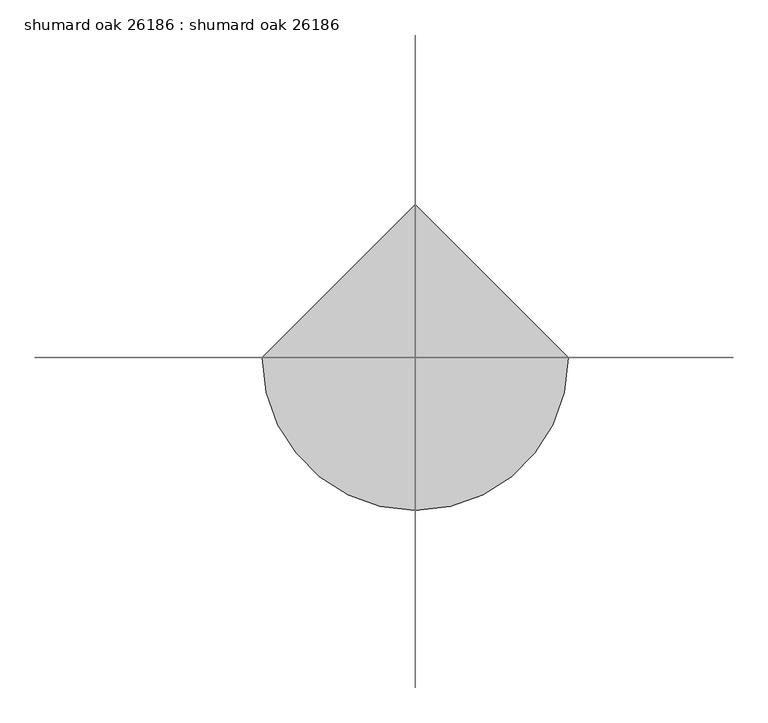
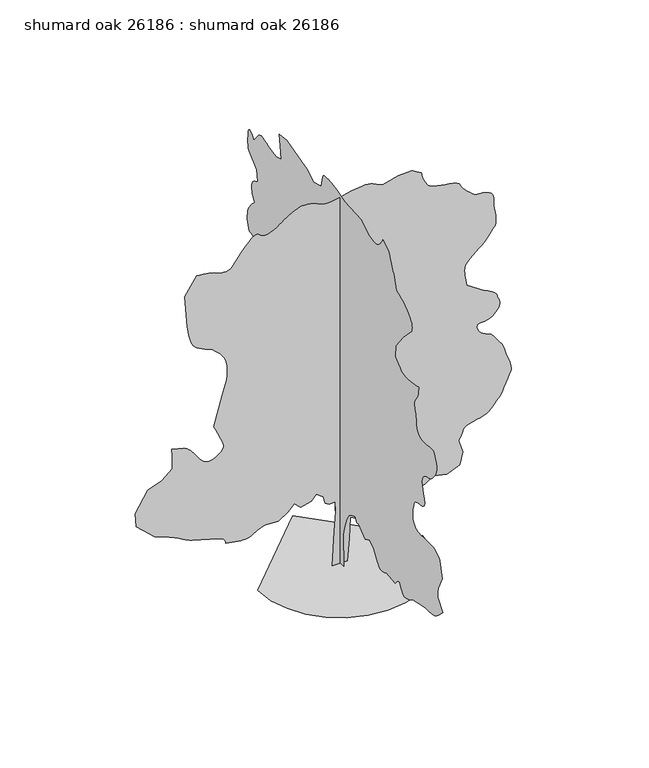
"""IFC4 building model written with IfcOpenShell, lengths in millimetres: proxy geometry, shumard oak 26186 : shumard oak 26186."""

import ifcopenshell
import ifcopenshell.guid

model = None  # the IFC model being written
_history = None  # IfcOwnerHistory: only IFC2X3 demands one
_inside = {}  # id of a spatial element -> (the spatial element, [elements in it])
_under = {}  # id of a project, library or spatial element -> (it, [spatial elements below it])
_declared = {}  # id of a project -> (the project, [libraries it declares])
_typed = {}  # id of a type object -> (the type object, [elements of that type])
_made_of = {}  # id of a material, layer set ... -> (it, [elements and type objects made of it])


def new_model(schema):
    """Start an empty IFC model of exactly this schema.

    Asked for "IFC4X3", IfcOpenShell would pick the latest addendum, in which some entities
    have other attributes; the version numbers below select the first issue.
    IFC2X3 requires an IfcOwnerHistory on every rooted entity: one is made here for all.
    """
    global model, _history
    if schema == "IFC4X3":
        model = ifcopenshell.file(schema_version=(4, 3, 0, 0))
    else:
        model = ifcopenshell.file(schema=schema)
    _inside.clear()
    _under.clear()
    _declared.clear()
    _typed.clear()
    _made_of.clear()
    _history = None
    if model.schema == "IFC2X3":
        org = make("IfcOrganization", Name="unknown")
        user = make(
            "IfcPersonAndOrganization",
            ThePerson=make("IfcPerson", FamilyName="unknown"),
            TheOrganization=org,
        )
        app = make(
            "IfcApplication",
            ApplicationDeveloper=org,
            Version="unknown",
            ApplicationFullName="unknown",
            ApplicationIdentifier="unknown",
        )
        _history = make(
            "IfcOwnerHistory",
            OwningUser=user,
            OwningApplication=app,
            ChangeAction="ADDED",
            CreationDate=0,
        )
    return model


def make(cls, **values):
    """One entity of the class cls with the attributes given. An attribute that is None is left unset."""
    return model.create_entity(
        cls, **{name: value for name, value in values.items() if value is not None}
    )


def rooted(cls, **values):
    """An entity with a GlobalId (a new one), such as an element, a storey or a relation."""
    return make(cls, GlobalId=ifcopenshell.guid.new(), OwnerHistory=_history, **values)


def si_unit(unit_type, name, prefix=None):
    """IfcSIUnit, for example si_unit("LENGTHUNIT", "METRE", prefix="MILLI")."""
    return make("IfcSIUnit", UnitType=unit_type, Prefix=prefix, Name=name)


def assignment(units):
    """IfcUnitAssignment: the units of a project."""
    return None if units is None else make("IfcUnitAssignment", Units=units)


def point(xyz):
    """IfcCartesianPoint."""
    return None if xyz is None else make("IfcCartesianPoint", Coordinates=xyz)


def direction(xyz):
    """IfcDirection."""
    return None if xyz is None else make("IfcDirection", DirectionRatios=xyz)


def frame(location, z_axis=None, x_axis=None):
    """IfcAxis2Placement3D, a coordinate frame: its origin and axes. An axis left out is left unset."""
    return make(
        "IfcAxis2Placement3D",
        Location=point(location),
        Axis=direction(z_axis),
        RefDirection=direction(x_axis),
    )


def origin():
    """The frame at (0, 0, 0) with its axes left unset."""
    return frame((0.0, 0.0, 0.0))


def place(relative_to, where):
    """IfcLocalPlacement: puts the frame where relative to a parent placement (None: the world)."""
    return make(
        "IfcLocalPlacement", PlacementRelTo=relative_to, RelativePlacement=where
    )


def context(
    kind, dimensions, precision=None, world=None, true_north=None, identifier=None
):
    """IfcGeometricRepresentationContext, for example the 3D "Model" context."""
    return make(
        "IfcGeometricRepresentationContext",
        ContextIdentifier=identifier,
        ContextType=kind,
        CoordinateSpaceDimension=dimensions,
        Precision=precision,
        WorldCoordinateSystem=world,
        TrueNorth=true_north,
    )


def project(units=None, contexts=None):
    """IfcProject with its units and contexts."""
    return rooted(
        "IfcProject",
        Name="project",
        RepresentationContexts=contexts,
        UnitsInContext=assignment(units),
    )


def spatial(cls, under=None, at=None, **own):
    """A site, building, storey or space (cls), placed at a placement, below another one or the project."""
    s = rooted(cls, ObjectPlacement=at, **own)
    if under is not None:
        _under.setdefault(under.id(), (under, []))[1].append(s)
    return s


def point_list(points):
    """IfcCartesianPointList2D or 3D."""
    cls = (
        "IfcCartesianPointList2D" if len(points[0]) == 2 else "IfcCartesianPointList3D"
    )
    return make(cls, CoordList=points)


def triangles(points, corners, closed=None, point_numbers=None):
    """IfcTriangulatedFaceSet: each triangle names its three corners, points numbered from 1."""
    return make(
        "IfcTriangulatedFaceSet",
        Coordinates=point_list(points),
        Closed=closed,
        CoordIndex=corners,
        PnIndex=point_numbers,
    )


def shape(context_of_items, identifier, shape_type, items):
    """IfcShapeRepresentation: the items that make up one representation, for example the "Body"."""
    return make(
        "IfcShapeRepresentation",
        ContextOfItems=context_of_items,
        RepresentationIdentifier=identifier,
        RepresentationType=shape_type,
        Items=items,
    )


def source(mapping_origin, context_of_items, identifier, shape_type, items):
    """IfcRepresentationMap: a shape defined once, which mapped items show again and again."""
    return make(
        "IfcRepresentationMap",
        MappingOrigin=mapping_origin,
        MappedRepresentation=shape(context_of_items, identifier, shape_type, items),
    )


def transform(
    local_origin,
    x_axis=None,
    y_axis=None,
    z_axis=None,
    scale=None,
    scale2=None,
    scale3=None,
    uniform=True,
):
    """IfcCartesianTransformationOperator3D, or its non-uniform kind. x_axis, y_axis, z_axis: its Axis1, 2, 3."""
    if uniform:
        return make(
            "IfcCartesianTransformationOperator3D",
            Axis1=direction(x_axis),
            Axis2=direction(y_axis),
            LocalOrigin=point(local_origin),
            Scale=scale,
            Axis3=direction(z_axis),
        )
    return make(
        "IfcCartesianTransformationOperator3DnonUniform",
        Axis1=direction(x_axis),
        Axis2=direction(y_axis),
        LocalOrigin=point(local_origin),
        Scale=scale,
        Axis3=direction(z_axis),
        Scale2=scale2,
        Scale3=scale3,
    )


def mapped(mapping_source, mapping_target):
    """IfcMappedItem: shows the shape of a source again, moved by a transform."""
    return make(
        "IfcMappedItem", MappingSource=mapping_source, MappingTarget=mapping_target
    )


def made_of(thing, what):
    """Note that an element or type object is made of a material, layer set ...; save() writes the relation."""
    if what is not None:
        _made_of.setdefault(what.id(), (what, []))[1].append(thing)
    return thing


def element(
    cls,
    number,
    at=None,
    inside=None,
    cuts=None,
    type_object=None,
    material=None,
    context=None,
    identifier="Body",
    shape_type=None,
    held_by="IfcProductDefinitionShape",
    body=None,
    shapes=None,
    **own,
):
    """One element of the class cls, such as IfcWall. Its Tag is "e" and its number.

    at: its placement. inside: the storey or other place that contains it. cuts: it is an
    opening in that element (IfcRelVoidsElement). A single representation is given by context,
    identifier, shape_type and body (its items); several are given by shapes. held_by: the class
    of the entity that holds the representations. save() writes the other relations.
    """
    e = rooted(cls, Tag="e%d" % number, ObjectPlacement=at, **own)
    if body is not None:
        shapes = [shape(context, identifier, shape_type, body)]
    if shapes is not None:
        e.Representation = make(held_by, Representations=shapes)
    if inside is not None:
        _inside.setdefault(inside.id(), (inside, []))[1].append(e)
    if cuts is not None:
        rooted(
            "IfcRelVoidsElement", RelatingBuildingElement=cuts, RelatedOpeningElement=e
        )
    if type_object is not None:
        _typed.setdefault(type_object.id(), (type_object, []))[1].append(e)
    return made_of(e, material)


def aggregate(whole, parts):
    """IfcRelAggregates: a whole, such as a stair, and the parts it consists of."""
    return rooted("IfcRelAggregates", RelatingObject=whole, RelatedObjects=parts)


def save(model, path):
    """Write the relations noted so far, then the file.

    IfcRelAggregates (storeys below a building ...), IfcRelContainedInSpatialStructure (elements
    in a storey), IfcRelDefinesByType, IfcRelAssociatesMaterial and IfcRelDeclares: one each for
    every whole, place, type object, material and project.
    """
    for whole, parts in _under.values():
        aggregate(whole, parts)
    for where, things in _inside.values():
        rooted(
            "IfcRelContainedInSpatialStructure",
            RelatedElements=things,
            RelatingStructure=where,
        )
    for kind, things in _typed.values():
        rooted("IfcRelDefinesByType", RelatedObjects=things, RelatingType=kind)
    for what, things in _made_of.values():
        rooted("IfcRelAssociatesMaterial", RelatedObjects=things, RelatingMaterial=what)
    for by, libraries in _declared.values():
        rooted("IfcRelDeclares", RelatingContext=by, RelatedDefinitions=libraries)
    model.write(path)


def shumard_oak_26186_shumard_oak_26186_cf07c7db(model_context):
    return source(origin(), model_context, "Body", "Tessellation", [
        triangles([(-0.0016958, 164.6246354, 0.0086022), (-0.0016958, -151.6104316, 0.0086022), (-0.0016958, -124.1113561, 783.7227293), (-0.0016958, -179.1089983, 1017.4612965), (-0.0016958, -261.6049622, 1237.4509209), (-0.0016958, -357.8507226, 1388.6927067), (-0.0016958, -467.8454985, 1457.4403999), (-0.0016958, -605.3383779, 1512.436607), (-0.0016958, -660.3370193, 1388.6927067), (-0.0016958, -756.5828161, 1416.1908829), (-0.0016958, -866.5775557, 1306.195998), (-0.0016958, -1017.8194868, 1209.9502739), (-0.0016958, -1196.5619196, 1292.4469826), (-0.0016958, -1361.5527935, 1182.452243), (-0.0016958, -1471.5476784, 989.9607222), (-0.0016958, -1498.1643677, 951.9597713), (-0.0016958, -1525.3829098, 915.7621988), (-0.0016958, -1553.8031227, 883.1739264), (-0.0016958, -1584.0290394, 855.9959341), (-0.0016958, -1616.658007, 836.0340712), (-0.0016958, -1652.2942039, 825.0891724), (-0.0016958, -1691.5371574, 824.9697756), (-0.0016958, -1729.1774471, 831.662681), (-0.0016958, -1760.3255459, 839.8008471), (-0.0016958, -1786.0582775, 849.1404659), (-0.0016958, -1807.4654011, 859.4426714), (-0.0016958, -1825.6238857, 870.4663445), (-0.0016958, -1841.6182583, 881.9725462), (-0.0016958, -1856.5307201, 893.7149254), (-0.0016958, -2214.0131149, 852.4678791), (-0.0016958, -2249.2480282, 893.1561659), (-0.0016958, -2283.7616192, 930.4738735), (-0.0016958, -2316.8324203, 961.0605967), (-0.0016958, -2347.7391094, 981.54314), (-0.0016958, -2375.7578934, 988.5586275), (-0.0016958, -2400.1697754, 978.7389507), (-0.0016958, -2420.2535786, 948.7136032), (-0.0016958, -2440.416156, 905.5412384), (-0.0016958, -2465.389341, 860.9260838), (-0.0016958, -2494.9323051, 818.4750412), (-0.0016958, -2528.8058189, 781.7974108), (-0.0016958, -2566.7735596, 754.4999491), (-0.0016958, -2608.5820541, 740.1896307), (-0.0016958, -2653.9973053, 742.4730669), (-0.0016958, -2699.5395836, 755.8614212), (-0.0016958, -2742.1861084, 772.1352098), (-0.0016958, -2782.4196991, 790.8169184), (-0.0016958, -2820.7484642, 811.421402), (-0.0016958, -2857.6293526, 833.4686754), (-0.0016958, -2893.5448929, 856.475992), (-0.0016958, -2928.9779045, 879.96591), (-0.0016958, -3423.9482735, 976.2117067), (-0.0016958, -3485.6956673, 976.3335743), (-0.0016958, -3546.579451, 977.174366), (-0.0016958, -3605.7868835, 979.4603456), (-0.0016958, -3662.4543549, 983.9078939), (-0.0016958, -3715.7688332, 991.2459635), (-0.0016958, -3764.8925789, 1002.1882462), (-0.0016958, -3808.9361115, 1017.4612965), (-0.0016958, -3851.3797417, 1039.546649), (-0.0016958, -3896.0075409, 1069.5719965), (-0.0016958, -3942.4134293, 1106.2115479), (-0.0016958, -3990.2924835, 1148.1393665), (-0.0016958, -4039.2383331, 1194.0371464), (-0.0016958, -4088.8951859, 1242.5817123), (-0.0016958, -4138.9334106, 1292.4469826), (-0.0016958, -3946.4265564, 1512.436607), (-0.0016958, -3940.7114983, 1553.6455742), (-0.0016958, -3935.9362083, 1594.6132771), (-0.0016958, -3933.0916145, 1635.0983059), (-0.0016958, -3933.1169037, 1674.8646286), (-0.0016958, -3937.0032944, 1713.6657486), (-0.0016958, -3945.7152626, 1751.2679592), (-0.0016958, -3960.1934486, 1787.4247639), (-0.0016958, -4111.425206, 2103.6601124), (-0.0016958, -4015.1842781, 2488.640538), (-0.0016958, -4007.6405525, 2499.2628548), (-0.0016958, -3985.1869812, 2526.4815422), (-0.0016958, -3948.0776184, 2563.3191193), (-0.0016958, -3896.5156494, 2602.8164177), (-0.0016958, -3830.780127, 2637.9697952), (-0.0016958, -3751.1003975, 2661.820665), (-0.0016958, -3657.7046448, 2667.3831161), (-0.0016958, -3553.6406479, 2663.0650658), (-0.0016958, -3446.4524231, 2661.3634254), (-0.0016958, -3343.1000107, 2661.617189), (-0.0016958, -3250.5928665, 2663.0650658), (-0.0016958, -3175.8660324, 2664.970182), (-0.0016958, -3125.9298363, 2666.6718224), (-0.0016958, -3107.7178665, 2667.3831161), (-0.0016958, -3097.049913, 2674.6474983), (-0.0016958, -3069.5669975, 2695.1200859), (-0.0016958, -3031.9495262, 2726.9207611), (-0.0016958, -2990.9793526, 2768.0688309), (-0.0016958, -2953.3874611, 2816.7097572), (-0.0016958, -2925.9045456, 2870.8625565), (-0.0016958, -2915.2365921, 2928.622403), (-0.0016958, -2917.2431557, 2986.3310898), (-0.0016958, -2922.8564758, 3041.9064766), (-0.0016958, -2931.4672874, 3095.6529053), (-0.0016958, -2942.4907425, 3147.977037), (-0.0016958, -2955.3178665, 3199.2087936), (-0.0016958, -2969.3385223, 3249.7039673), (-0.0016958, -2983.9690247, 3299.8436394), (-0.0016958, -2996.0086967, 3314.52472), (-0.0016958, -3009.4706657, 3328.8250099), (-0.0016958, -3025.8280975, 3342.414006), (-0.0016958, -3046.5038704, 3354.9362068), (-0.0016958, -3072.9705688, 3365.9852417), (-0.0016958, -3106.6510712, 3375.2561874), (-0.0016958, -3148.9673836, 3382.3429642), (-0.0016958, -3200.1485619, 3386.6863037), (-0.0016958, -3255.4443146, 3391.740937), (-0.0016958, -3308.7843727, 3403.2725006), (-0.0016958, -3354.1996239, 3427.0722107), (-0.0016958, -3385.6703773, 3468.9315742), (-0.0016958, -3397.1766518, 3534.5906479), (-0.0016958, -3382.6984657, 3629.8406479), (-0.0016958, -3353.0819595, 3737.5114014), (-0.0016958, -3325.8786781, 3836.2667107), (-0.0016958, -3305.152327, 3925.6746254), (-0.0016958, -3294.9921913, 4005.2023293), (-0.0016958, -3299.5387161, 4074.3920013), (-0.0016958, -3322.8306084, 4132.761113), (-0.0016958, -3368.9571533, 4179.8018463), (-0.0016958, -3425.5228867, 4212.7710548), (-0.0016958, -3477.9993347, 4232.964299), (-0.0016958, -3527.3262657, 4246.1975029), (-0.0016958, -3574.5193153, 4258.2118858), (-0.0016958, -3620.493544, 4274.8233719), (-0.0016958, -3666.2390076, 4301.7473099), (-0.0016958, -3712.6954742, 4344.8004959), (-0.0016958, -3760.0411308, 4399.562851), (-0.0016958, -3805.2023277, 4457.9322533), (-0.0016958, -3844.3694138, 4520.1368866), (-0.0016958, -3873.6809967, 4586.4308052), (-0.0016958, -3889.2765564, 4657.068354), (-0.0016958, -3887.295282, 4732.2777168), (-0.0016958, -3863.9272316, 4812.2879494), (-0.0016958, -3835.7077332, 4887.9545517), (-0.0016958, -3816.632444, 4949.7019455), (-0.0016958, -3799.0047409, 4996.9967331), (-0.0016958, -3775.1032928, 5029.3819656), (-0.0016958, -3737.2573471, 5046.3745331), (-0.0016958, -3677.7705711, 5047.4919067), (-0.0016958, -3588.9466324, 5032.2771378), (-0.0016958, -3483.5620766, 5015.437468), (-0.0016958, -3382.266806, 5012.0591858), (-0.0016958, -3289.150106, 5022.1684525), (-0.0016958, -3208.3018433, 5045.7396881), (-0.0016958, -3143.7860138, 5082.7728928), (-0.0016958, -3099.7421906, 5133.2930649), (-0.0016958, -3080.2096619, 5197.2507889), (-0.0016958, -3073.5295464, 5265.5768509), (-0.0016958, -3065.4015541, 5329.5339935), (-0.0016958, -3056.0541595, 5389.9099594), (-0.0016958, -3045.7417076, 5447.3901718), (-0.0016958, -3034.7182526, 5502.7112137), (-0.0016958, -3023.2119781, 5556.5846695), (-0.0016958, -3011.4772293, 5609.7471222), (-0.0016958, -3000.047113, 5648.0755966), (-0.0016958, -2990.8014565, 5686.505809), (-0.0016958, -2985.8485611, 5725.1900757), (-0.0016958, -2987.423465, 5764.2295532), (-0.0016958, -2997.6341789, 5803.7521408), (-0.0016958, -3018.6907425, 5843.8839935), (-0.0016958, -3052.7267464, 5884.7274307), (-0.0016958, -3089.125106, 5934.8418137), (-0.0016958, -3116.6080215, 5997.6815826), (-0.0016958, -3136.4198936, 6065.8297485), (-0.0016958, -3149.7295464, 6131.8187439), (-0.0016958, -3157.7558006, 6188.1815826), (-0.0016958, -3161.6674805, 6227.450116), (-0.0016958, -3162.7089867, 6242.2073547), (-0.0016958, -3142.4395844, 6237.6861191), (-0.0016958, -3088.0074417, 6226.1798447), (-0.0016958, -3009.0387154, 6210.8383392), (-0.0016958, -2915.160434, 6194.7602509), (-0.0016958, -2815.9731743, 6181.0948059), (-0.0016958, -2721.1295448, 6172.9418152), (-0.0016958, -2640.2304131, 6173.4749222), (-0.0016958, -2571.9299309, 6185.3619873), (-0.0016958, -2507.9599983, 6208.094902), (-0.0016958, -2447.5915901, 6239.8452896), (-0.0016958, -2390.1089069, 6278.808609), (-0.0016958, -2334.7901905, 6323.1826447), (-0.0016958, -2280.9167347, 6371.1634369), (-0.0016958, -2227.7621304, 6420.9476074), (-0.0016958, -2241.5111458, 6709.6945175), (-0.0016958, -2543.9897758, 7094.6826462), (-0.0016958, -2887.7283875, 7452.1625702), (-0.0016958, -2893.1132332, 7496.4860275), (-0.0016958, -2895.3482712, 7541.6722229), (-0.0016958, -2891.335144, 7588.5356415), (-0.0016958, -2877.9493332, 7637.9128601), (-0.0016958, -2852.0666107, 7690.6689423), (-0.0016958, -2810.5377502, 7747.6160477), (-0.0016958, -2750.2379425, 7809.6424942), (-0.0016958, -2679.5242355, 7869.2562973), (-0.0016958, -2608.8108192, 7919.4724182), (-0.0016958, -2538.10467, 7961.8901779), (-0.0016958, -2467.3935791, 7998.0344833), (-0.0016958, -2396.6824883, 8029.5052368), (-0.0016958, -2325.9712521, 8057.8517624), (-0.0016958, -2255.2601612, 8084.6233841), (-0.0016958, -2234.6175259, 8155.1336151), (-0.0016958, -2213.8530956, 8224.4503143), (-0.0016958, -2192.8472557, 8291.3537888), (-0.0016958, -2171.4808273, 8354.651088), (-0.0016958, -2149.6341957, 8413.1219376), (-0.0016958, -2127.1881821, 8465.5983856), (-0.0016958, -2104.0183754, 8510.8607391), (-0.0016958, -2078.3235775, 8560.2129593), (-0.0016958, -2049.9822842, 8621.0970337), (-0.0016958, -2021.4021973, 8686.5529221), (-0.0016958, -1994.9862225, 8749.5955856), (-0.0016958, -1973.1395908, 8803.2917267), (-0.0016958, -1958.2679695, 8840.6039841), (-0.0016958, -1952.7738281, 8854.5996414), (-0.0016958, -1719.0353336, 8992.089505), (-0.0016958, -1707.0516174, 8968.3915329), (-0.0016958, -1693.863905, 8943.9819763), (-0.0016958, -1678.2681999, 8918.1248337), (-0.0016958, -1659.0683544, 8890.1085205), (-0.0016958, -1635.057756, 8859.1970352), (-0.0016958, -1605.0324085, 8824.678212), (-0.0016958, -1567.7934025, 8785.841629), (-0.0016958, -1522.9369835, 8752.2122864), (-0.0016958, -1471.5882282, 8732.2983856), (-0.0016958, -1414.8268673, 8723.7896027), (-0.0016958, -1353.7372822, 8724.4244476), (-0.0016958, -1289.3990582, 8731.9175949), (-0.0016958, -1222.896722, 8743.9825562), (-0.0016958, -1155.3123299, 8758.3334244), (-0.0016958, -852.8259968, 8964.5813004), (-0.0016958, -192.8582863, 9005.8311081), (-0.0016958, -107.5965211, 9029.2756073), (-0.0016958, -23.416737, 9052.008522), (-0.0016958, 58.5983536, 9073.2938507), (-0.0016958, 137.366361, 9092.4200089), (-0.0016958, 211.8051857, 9108.6504135), (-0.0016958, 280.8327856, 9121.2740616), (-0.0016958, 343.3650879, 9129.57995), (-0.0016958, 405.0185557, 9135.9045639), (-0.0016958, 469.5549508, 9141.5181747), (-0.0016958, 533.1311937, 9144.0075577), (-0.0016958, 591.8966838, 9140.9594879), (-0.0016958, 642.0033274, 9129.9863205), (-0.0016958, 679.6029219, 9108.6504135), (-0.0016958, 700.8500261, 9074.5891205), (-0.0016958, 769.5952486, 8799.5832321), (-0.0016958, 1072.081509, 8717.1091965), (-0.0016958, 1347.0698112, 8882.0822662), (-0.0016958, 1690.8031906, 8964.5813004), (-0.0016958, 2144.5313095, 9102.0717453), (-0.0016958, 2447.0174973, 9060.8225189), (-0.0016958, 2419.5169956, 8799.5832321), (-0.0016958, 2364.5209339, 8497.1197174), (-0.0016958, 2584.5030006, 8428.361705), (-0.0016958, 2804.4924797, 8469.6115128), (-0.0016958, 2889.5570549, 8501.5647949), (-0.0016958, 2972.3357231, 8530.7490601), (-0.0016958, 3050.5425774, 8554.3964539), (-0.0016958, 3121.8911293, 8569.7385406), (-0.0016958, 3184.1210518, 8574.0307205), (-0.0016958, 3234.8958595, 8564.480722), (-0.0016958, 3271.9799332, 8538.3439453), (-0.0016958, 3478.2280998, 8290.8712601), (-0.0016958, 3525.090937, 8345.6591949), (-0.0016958, 3570.2521339, 8393.3603531), (-0.0016958, 3612.0606285, 8426.8885391), (-0.0016958, 3648.8144897, 8439.1058167), (-0.0016958, 3678.8373665, 8422.9515701), (-0.0016958, 3700.4526169, 8371.313443), (-0.0016958, 3711.9588913, 8277.1046585), (-0.0016958, 3715.4389114, 8172.4819748), (-0.0016958, 3714.6005905, 8091.684581), (-0.0016958, 3710.155513, 8030.6987686), (-0.0016958, 3702.8149727, 7985.6137299), (-0.0016958, 3693.3152618, 7952.4163376), (-0.0016958, 3682.3679649, 7927.1684601), (-0.0016958, 3670.7093742, 7905.8831314), (-0.0016958, 3354.4789673, 7644.6438446), (-0.0016958, 3326.9707626, 7355.921933), (-0.0016958, 3370.9384277, 7337.989888), (-0.0016958, 3413.6102417, 7318.6346741), (-0.0016958, 3453.615358, 7296.384288), (-0.0016958, 3489.6326363, 7269.8161423), (-0.0016958, 3520.3920959, 7237.4564896), (-0.0016958, 3544.5220184, 7197.8833237), (-0.0016958, 3560.7018448, 7149.674057), (-0.0016958, 3566.8994316, 7096.6389221), (-0.0016958, 3562.9624626, 7043.6032059), (-0.0016958, 3550.618158, 6990.568071), (-0.0016958, 3531.5425781, 6937.5329361), (-0.0016958, 3507.4126556, 6884.4978012), (-0.0016958, 3479.904451, 6831.4626663), (-0.0016958, 3450.7198952, 6778.4269501), (-0.0016958, 3494.7381386, 6734.2313919), (-0.0016958, 3537.6640068, 6689.8829361), (-0.0016958, 3578.4309952, 6645.3060059), (-0.0016958, 3615.9470192, 6600.3732834), (-0.0016958, 3649.1447021, 6554.9580322), (-0.0016958, 3676.9322502, 6508.9329346), (-0.0016958, 3698.2175789, 6462.1968338), (-0.0016958, 3713.4829262, 6416.6548462), (-0.0016958, 3724.4305138, 6374.0080307), (-0.0016958, 3731.7710541, 6333.77444), (-0.0016958, 3736.2161316, 6295.4459656), (-0.0016958, 3738.5020386, 6258.5650772), (-0.0016958, 3739.3400688, 6222.6492462), (-0.0016958, 3739.4670959, 6187.2165253), (-0.0016958, 3656.9680618, 5953.4854431), (-0.0016958, 3618.6901657, 5947.3387253), (-0.0016958, 3580.5140076, 5939.7694199), (-0.0016958, 3542.591613, 5929.304361), (-0.0016958, 3505.0250107, 5914.5215424), (-0.0016958, 3467.9665169, 5893.9477982), (-0.0016958, 3431.4664192, 5866.1599594), (-0.0016958, 3395.728775, 5829.7366013), (-0.0016958, 3363.165937, 5786.4799393), (-0.0016958, 3335.6830215, 5739.6171021), (-0.0016958, 3312.3911293, 5689.7567734), (-0.0016958, 3292.4522301, 5637.4838013), (-0.0016958, 3275.0532921, 5583.4068695), (-0.0016958, 3259.3559944, 5528.1364059), (-0.0016958, 3244.4717285, 5472.2566772), (-0.0016958, 3212.2896812, 5428.0349579), (-0.0016958, 3181.4287743, 5383.7120819), (-0.0016958, 3153.2092758, 5339.1351517), (-0.0016958, 3128.9523262, 5294.1768494), (-0.0016958, 3110.0037735, 5248.7615982), (-0.0016958, 3097.6341797, 5202.7620804), (-0.0016958, 3093.2399712, 5156.026561), (-0.0016958, 3106.9812836, 4784.7797447), (-0.0016958, 3139.1630402, 4781.5284897), (-0.0016958, 3170.049527, 4776.4738564), (-0.0016958, 3198.2690254, 4767.8377556), (-0.0016958, 3222.5006859, 4753.7662308), (-0.0016958, 3241.4745277, 4732.4809021), (-0.0016958, 3253.8188324, 4702.1533928), (-0.0016958, 3258.2383301, 4661.0306122), (-0.0016958, 3257.0192184, 4613.5073502), (-0.0016958, 3253.6665161, 4565.2219254), (-0.0016958, 3248.4848557, 4516.377523), (-0.0016958, 3241.8808983, 4467.0253029), (-0.0016958, 3234.1845657, 4417.3175812), (-0.0016958, 3225.7516502, 4367.3810944), (-0.0016958, 3216.988813, 4317.2922913), (-0.0016958, 3203.2219208, 4042.311692), (-0.0016958, 3464.4612076, 4056.0785843), (-0.0016958, 3753.208699, 4111.0694138), (-0.0016958, 3814.6511696, 4090.2669044), (-0.0016958, 3873.5792587, 4068.37202), (-0.0016958, 3927.4527145, 4044.3182556), (-0.0016958, 3973.7568649, 4017.0132362), (-0.0016958, 4009.9520393, 3985.3901665), (-0.0016958, 4033.523275, 3948.3569618), (-0.0016958, 4041.9306107, 3904.8212471), (-0.0016958, 4039.5429657, 3849.6778107), (-0.0016958, 4032.8119812, 3780.081768), (-0.0016958, 4022.448951, 3698.4716331), (-0.0016958, 4009.2407455, 3607.2347603), (-0.0016958, 3993.8483711, 3508.7840836), (-0.0016958, 3977.00812, 3405.5078293), (-0.0016958, 3959.4568657, 3299.8436394), (-0.0016958, 3835.7077332, 2969.87192), (-0.0016958, 3768.1185448, 2931.9498161), (-0.0016958, 3701.6211502, 2896.3136192), (-0.0016958, 3637.2829262, 2865.2492363), (-0.0016958, 3576.1959572, 2841.0431557), (-0.0016958, 3519.4267479, 2825.9554138), (-0.0016958, 3468.0679642, 2822.3233681), (-0.0016958, 3423.2113998, 2832.3817657), (-0.0016958, 3038.248851, 2997.3548355), (-0.0016958, 2653.2607224, 2873.6312828), (-0.0016958, 2378.2699493, 2681.1244286), (-0.0016958, 2103.2842632, 2268.651059), (-0.0016958, 2076.6675739, 2227.6428062), (-0.0016958, 2049.4488865, 2188.0796688), (-0.0016958, 2021.0263481, 2151.4021111), (-0.0016958, 1990.8027569, 2119.0526321), (-0.0016958, 1958.1739346, 2092.4764927), (-0.0016958, 1922.5377377, 2073.1141571), (-0.0016958, 1883.2946388, 2062.4105953), (-0.0016958, 1844.1303143, 2058.8443886), (-0.0016958, 1807.3715115, 2059.123732), (-0.0016958, 1770.371299, 2062.0498615), (-0.0016958, 1730.4881229, 2066.4186356), (-0.0016958, 1685.070401, 2071.0288193), (-0.0016958, 1631.4762886, 2074.6762711), (-0.0016958, 1567.0592903, 2076.1596107), (-0.0016958, 1497.9510086, 2070.950045), (-0.0016958, 1431.730632, 2056.3577671), (-0.0016958, 1367.9130157, 2033.9498325), (-0.0016958, 1306.020718, 2005.2883553), (-0.0016958, 1245.5712101, 1971.9382107), (-0.0016958, 1186.0844341, 1935.4612221), (-0.0016958, 1127.0801868, 1897.4196487), (-0.0016958, 1044.5834782, 1663.6810089), (-0.0016958, 810.8448383, 1402.4418674), (-0.0016958, 778.5741337, 1367.4862976), (-0.0016958, 741.256426, 1333.2546661), (-0.0016958, 699.7273476, 1299.622562), (-0.0016958, 654.8303061, 1266.4729866), (-0.0016958, 607.408455, 1233.6815289), (-0.0016958, 558.3051295, 1201.1339516), (-0.0016958, 508.3585416, 1168.7032276), (-0.0016958, 425.8618329, 1457.4403999), (-0.0016958, 288.3689717, 1649.9293774), (-0.0016958, 233.3715837, 1526.1856224), (-0.0016958, 192.1232112, 1333.696645), (-0.0016958, 178.3741776, 989.9607222), (-0.0016958, 150.8753565, 508.7344634), (170.3625119, 0.000436, 0.0217742), (-187.1199193, 0.000436, 0.0217742), (-132.1230309, 0.000387, 824.9824928), (-104.6242098, 0.0003581, 1306.2087879), (-118.3734886, 0.0003434, 1553.698914), (-255.8671038, 0.0003442, 1539.9498985), (-352.1128461, 0.000341, 1594.9459602), (-393.359965, 0.0003302, 1773.6885384), (-558.3534187, 0.0003237, 1883.6832779), (-668.3482309, 0.000331, 1759.9395229), (-915.8358135, 0.0003352, 1691.1918297), (-1067.0802881, 0.0003271, 1828.6846001), (-1218.3221466, 0.000336, 1677.4428143), (-1438.311771, 0.0003442, 1539.9498985), (-1768.2961349, 0.0003434, 1553.698914), (-1933.2869362, 0.0003476, 1484.9512207), (-1968.7250347, 0.0003491, 1458.6138748), (-2004.6407204, 0.0003507, 1433.3612011), (-2041.5189926, 0.000352, 1410.2726395), (-2079.8425255, 0.0003531, 1390.4301006), (-2120.0889061, 0.0003541, 1374.915786), (-2162.738047, 0.0003547, 1364.8142223), (-2208.2752384, 0.0003549, 1361.2074657), (-2259.0244663, 0.0003549, 1362.8101295), (-2316.2658852, 0.0003547, 1367.3008438), (-2378.9175842, 0.0003541, 1374.1944637), (-2445.902449, 0.0003536, 1383.0132568), (-2516.1310112, 0.0003531, 1393.2749851), (-2588.5161278, 0.0003523, 1404.4991547), (-2661.9982704, 0.0003518, 1416.2061436), (-2665.4018417, 0.0003499, 1445.5887978), (-2671.5741394, 0.0003481, 1474.4889233), (-2683.2835991, 0.0003465, 1502.428933), (-2703.2986565, 0.0003449, 1528.9262981), (-2734.3630394, 0.0003434, 1553.4981995), (-2779.2448929, 0.0003421, 1575.6648697), (-2840.7382324, 0.000341, 1594.9459602), (-3445.7158401, 0.0003302, 1773.6885384), (-3495.0936401, 0.0003295, 1789.3602562), (-3547.8494316, 0.0003281, 1811.5293972), (-3602.2815742, 0.0003266, 1838.265556), (-3656.7140076, 0.0003247, 1867.6482101), (-3709.469799, 0.0003229, 1897.7523319), (-3758.8728882, 0.0003213, 1926.6550735), (-3803.1957642, 0.0003197, 1952.4285004), (-3850.8716331, 0.0003182, 1977.2011162), (-3910.0790657, 0.0003166, 2004.1403149), (-3978.8876564, 0.0003148, 2032.8804211), (-4055.4181595, 0.0003132, 2063.0657879), (-4137.7140083, 0.0003113, 2094.3332108), (-4223.8456696, 0.0003092, 2126.3194851), (-4311.9327347, 0.0003074, 2158.668964), (-4738.1450912, 0.0002835, 2557.4011665), (-4765.6532959, 0.0002638, 2887.3725952), (-4476.9060951, 0.000236, 3354.8600487), (-4146.9343758, 0.0002287, 3478.6088905), (-3899.4364014, 0.0002163, 3684.8570572), (-3899.4364014, 0.0001977, 4001.0874641), (-3913.2032936, 0.0001877, 4166.0858231), (-3624.4558022, 0.0001919, 4097.3281013), (-3591.9438332, 0.0001932, 4076.3729851), (-3558.8475975, 0.0001945, 4053.3607269), (-3524.5322502, 0.0001961, 4026.2588928), (-3488.4135246, 0.0001979, 3993.03563), (-3449.8815742, 0.0002006, 3951.6082169), (-3408.3524231, 0.0002037, 3899.9953789), (-3363.216806, 0.0002074, 3836.0888145), (-3317.4713425, 0.0002113, 3768.956575), (-3273.4275192, 0.000215, 3709.7491425), (-3229.3839867, 0.0002179, 3659.6856285), (-3183.6385231, 0.0002203, 3619.9601463), (-3134.5403572, 0.0002221, 3591.765937), (-3080.387558, 0.0002229, 3576.3482735), (-3019.4781944, 0.0002229, 3574.8495277), (-2952.9046417, 0.0002221, 3590.0895859), (-2885.848851, 0.0002203, 3620.9507835), (-2822.8567657, 0.0002176, 3662.8860146), (-2768.5513596, 0.0002147, 3711.2984665), (-2727.4541588, 0.0002119, 3761.6413239), (-2704.1622665, 0.000209, 3809.3427727), (-2703.2480782, 0.0002066, 3849.8304176), (-2719.4531937, 0.000204, 3893.6198959), (-2743.5831161, 0.0002006, 3952.5479851), (-2774.3172867, 0.0001961, 4024.0997223), (-2810.3598541, 0.0001914, 4105.735437), (-2850.3649704, 0.0001861, 4194.9657463), (-2893.0114952, 0.0001803, 4289.2506889), (-2936.9788696, 0.0001746, 4386.0755928), (-2744.4975952, 0.0001328, 5087.2685486), (-2718.1576332, 0.0001281, 5166.6433548), (-2692.9100464, 0.0001234, 5244.9263672), (-2669.8216301, 0.0001189, 5321.050209), (-2649.9841782, 0.0001145, 5393.948085), (-2634.4647766, 0.0001105, 5462.477623), (-2624.3555099, 0.0001066, 5525.6220245), (-2620.7487534, 0.0001034, 5582.263916), (-2621.6885216, 0.0001, 5637.5343796), (-2624.7618805, 9.66e-05, 5696.1831253), (-2630.5022278, 9.29e-05, 5756.5079315), (-2639.366803, 8.93e-05, 5816.8333191), (-2651.8128456, 8.58e-05, 5875.4820648), (-2668.3737534, 8.24e-05, 5930.7525284), (-2689.5064751, 7.95e-05, 5980.9936478), (-2716.6844673, 7.67e-05, 6027.7297485), (-2750.3649696, 7.4e-05, 6073.7542648), (-2789.4303177, 7.14e-05, 6119.169516), (-2832.8390053, 6.85e-05, 6164.1022385), (-2879.4986572, 6.59e-05, 6208.6791687), (-2928.3430595, 6.33e-05, 6253.002626), (-2978.2286774, 6.06e-05, 6297.223764), (-3057.4511673, 5.88e-05, 6329.6851547), (-3134.6165154, 5.67e-05, 6362.5273361), (-3207.6922874, 5.49e-05, 6396.0805206), (-3274.6213417, 5.28e-05, 6430.7010818), (-3333.3971146, 5.07e-05, 6466.7942276), (-3381.9365936, 4.83e-05, 6504.6657532), (-3418.2076355, 4.59e-05, 6544.7214478), (-3446.7573463, 4.28e-05, 6598.1123749), (-3473.1478867, 3.86e-05, 6670.5027237), (-3496.8717293, 3.36e-05, 6753.9668152), (-3517.4710533, 2.84e-05, 6840.5557159), (-3534.4636208, 2.34e-05, 6922.3181671), (-3547.3669029, 1.94e-05, 6991.3558136), (-3555.7233696, 1.65e-05, 7039.6918167), (-3610.7144897, -2.94e-05, 7809.6424942), (-3335.7086014, -5.49e-05, 8235.8804306), (-3262.2517479, -5.43e-05, 8226.9396973), (-3189.8616898, -5.38e-05, 8217.4146973), (-3119.6305115, -5.3e-05, 8206.6705856), (-3052.6252991, -5.22e-05, 8194.1225143), (-2989.9887154, -5.15e-05, 8179.162381), (-2932.7372681, -5.04e-05, 8161.2041748), (-2881.9880402, -4.91e-05, 8139.6397934), (-2830.4004913, -4.78e-05, 8118.7864151), (-2772.3107231, -4.7e-05, 8104.2064911), (-2711.3504906, -4.65e-05, 8097.069136), (-2651.1018425, -4.67e-05, 8098.5934616), (-2595.1709541, -4.73e-05, 8109.9724182), (-2547.1901619, -4.86e-05, 8132.4262802), (-2510.7589554, -5.07e-05, 8167.1224182), (-2290.7694763, -6.8e-05, 8455.8699097), (-2232.0038773, -7.19e-05, 8523.1291763), (-2174.2011555, -7.59e-05, 8587.3915329), (-2118.3236069, -7.93e-05, 8645.6333267), (-2065.3290218, -8.22e-05, 8694.8588104), (-2016.1850739, -8.45e-05, 8732.0699112), (-1971.8492626, -8.58e-05, 8754.2185593), (-1933.2869362, -8.61e-05, 8758.3590042), (-1902.260923, -8.53e-05, 8748.0212631), (-1877.0081039, -8.43e-05, 8731.181012), (-1853.1982201, -8.32e-05, 8711.4450073), (-1826.5002857, -8.22e-05, 8692.4455856), (-1792.5886929, -8.11e-05, 8677.7900848), (-1747.1302757, -8.09e-05, 8671.0591003), (-1685.7992809, -8.11e-05, 8675.8593887), (-1612.5227943, -8.24e-05, 8696.712767), (-1537.32346, -8.43e-05, 8731.5112244), (-1465.0070892, -8.69e-05, 8773.9795624), (-1400.3895218, -8.95e-05, 8817.9216476), (-1348.2787491, -9.19e-05, 8857.0378647), (-1313.4833439, -9.35e-05, 8885.1047562), (-1300.8163845, -9.42e-05, 8895.8488678), (-1285.3045406, -9.48e-05, 8905.7802383), (-1244.0574944, -9.63e-05, 8931.6123825), (-1185.0100084, -9.84e-05, 8967.2741592), (-1116.1022959, -0.0001008, 9006.7961655), (-1045.2718082, -0.0001029, 9044.1595825), (-980.4534536, -0.0001047, 9073.344429), (-929.5848289, -0.0001055, 9088.3307236), (-881.3222952, -0.0001058, 9091.6578461), (-821.2740709, -0.0001058, 9089.7021515), (-752.8083372, -0.0001053, 9082.2090042), (-679.2905136, -0.0001045, 9068.9505112), (-604.0912156, -0.0001034, 9049.6714554), (-530.573392, -0.0001019, 9024.1189453), (-462.1076583, -0.0001, 8992.089505), (-389.2730779, -9.84e-05, 8965.9533096), (-302.0062388, -9.79e-05, 8956.4283096), (-202.713753, -9.79e-05, 8960.7204895), (-93.8012603, -9.9e-05, 8976.0625763), (22.3266441, -0.0001003, 8999.7099701), (143.2647473, -0.0001021, 9028.8942352), (266.608781, -0.000104, 9060.8475174), (351.7496415, -0.0001047, 9072.3793716), (435.0871056, -0.0001053, 9082.4886383), (514.8177767, -0.0001058, 9089.7021515), (589.1356968, -0.0001058, 9092.597905), (656.2400311, -0.0001058, 9089.7021515), (714.324785, -0.000105, 9079.5928848), (761.584037, -0.000104, 9060.8475174), (801.2284195, -0.0001026, 9038.8767654), (837.987295, -0.0001016, 9019.8011856), (872.3408667, -0.0001005, 9003.1132507), (904.7690472, -9.98e-05, 8988.356012), (935.7570539, -9.9e-05, 8975.0719391), (965.779858, -9.82e-05, 8962.7017639), (995.3226768, -9.74e-05, 8950.8402786), (1352.8050716, -0.0001032, 9047.0809158), (1669.0404202, -0.000104, 9060.8475174), (1889.0325153, -9.66e-05, 8937.0986755), (1892.1974384, -9.48e-05, 8904.5611267), (1896.6881527, -9.27e-05, 8871.1602585), (1903.8228916, -9.06e-05, 8836.0827484), (1914.9278824, -8.85e-05, 8798.4908569), (1931.3210678, -8.58e-05, 8757.5206833), (1954.3308552, -8.32e-05, 8712.3339066), (1985.2757687, -8.03e-05, 8662.118367), (2016.3831722, -7.74e-05, 8616.1438477), (2042.1971489, -7.56e-05, 8582.1842926), (2067.531213, -7.4e-05, 8557.1398911), (2097.1958267, -7.27e-05, 8537.8358368), (2135.9969467, -7.19e-05, 8521.1990616), (2188.7502674, -7.09e-05, 8504.1047562), (2260.2639256, -6.96e-05, 8483.3781143), (2348.4121788, -6.85e-05, 8463.4136353), (2443.5351517, -6.75e-05, 8448.2500259), (2539.1383278, -6.67e-05, 8434.3055283), (2628.7244293, -6.56e-05, 8417.9478058), (2705.8133286, -6.43e-05, 8395.5701019), (2763.9030968, -6.25e-05, 8363.5918213), (2796.4915146, -5.99e-05, 8318.3794647), (2820.5705681, -5.67e-05, 8265.7507004), (2856.206765, -5.36e-05, 8213.8329391), (2901.4696999, -5.04e-05, 8162.5250244), (2954.4286766, -4.75e-05, 8111.6996384), (3013.1535805, -4.44e-05, 8061.2300446), (3075.7137154, -4.15e-05, 8011.0139236), (3140.2298355, -3.83e-05, 7960.8995407), (3230.9333107, -3.78e-05, 7951.6035965), (3317.928582, -3.73e-05, 7939.5386353), (3397.4559952, -3.62e-05, 7921.9362213), (3465.8073463, -3.47e-05, 7896.027919), (3519.2235626, -3.23e-05, 7859.0708725), (3554.0217293, -2.94e-05, 7808.2966461), (3566.4421921, -2.55e-05, 7740.9100616), (3567.2549332, -2.13e-05, 7670.7044632), (3569.4902618, -1.76e-05, 7612.0812973), (3572.9447021, -1.47e-05, 7563.0337097), (3577.3641998, -1.23e-05, 7521.7077438), (3582.4949913, -1.02e-05, 7486.1732849), (3588.1086021, -8.1e-06, 7454.4484772), (3593.9503967, -6.6e-06, 7424.6799454), (3605.4566711, -2.4e-06, 7354.1947128), (3615.2865944, 1.8e-06, 7285.1832275), (3621.7382355, 5.8e-06, 7219.0413345), (3623.1352432, 9.5e-06, 7157.2177826), (3617.8009758, 1.29e-05, 7101.1851563), (3604.0596634, 1.58e-05, 7052.3666245), (3580.2090843, 1.81e-05, 7012.1836121), (3549.779837, 2.05e-05, 6973.6772415), (3516.9376556, 2.31e-05, 6929.6084198), (3480.9965355, 2.6e-05, 6881.221257), (3441.1948952, 2.89e-05, 6829.7098663), (3396.8208595, 3.2e-05, 6776.2933594), (3347.138427, 3.54e-05, 6722.1408508), (3291.4615929, 3.86e-05, 6668.4452911), (3226.8184456, 4.2e-05, 6613.0986694), (3154.6824417, 4.54e-05, 6553.8912369), (3081.1241409, 4.91e-05, 6492.0421051), (3012.1376541, 5.28e-05, 6428.7453873), (2953.7429626, 5.67e-05, 6365.2196136), (2911.9344681, 6.04e-05, 6302.6338989), (2892.7321518, 6.41e-05, 6242.2329346), (2889.6587929, 6.75e-05, 6182.4918137), (2891.6144875, 7.11e-05, 6121.3286865), (2897.7867851, 7.48e-05, 6058.9464478), (2907.3370743, 7.88e-05, 5995.6241501), (2919.4020355, 8.24e-05, 5931.5652695), (2933.1436386, 8.64e-05, 5867.0238602), (2947.7232719, 9.03e-05, 5802.2533951), (3360.2196053, 0.0001066, 5527.2475067), (3376.1959557, 0.0001071, 5520.1357315), (3417.4457634, 0.0001082, 5500.475885), (3473.8591805, 0.00011, 5470.9864059), (3535.3019417, 0.0001121, 5434.2584152), (3591.7153587, 0.0001147, 5392.9830276), (3632.9648758, 0.0001171, 5349.7525269), (3648.9415169, 0.0001197, 5307.2580276), (3657.5267487, 0.0001221, 5267.1511734), (3677.1610153, 0.0001244, 5227.0193207), (3698.7256874, 0.0001271, 5183.5347656), (3713.0765556, 0.0001302, 5133.2930649), (3711.0699921, 0.0001336, 5072.9682587), (3683.5870766, 0.0001381, 4999.1814835), (3621.4586014, 0.0001436, 4908.5282959), (3535.7588905, 0.0001481, 4831.4141075), (3447.6462456, 0.0001504, 4791.5613075), (3363.1403572, 0.0001515, 4775.7881424), (3288.2612068, 0.0001517, 4770.8096672), (3229.0029053, 0.0001523, 4763.4182579), (3191.4110138, 0.0001536, 4740.4312889), (3181.4796432, 0.0001567, 4688.5388168), (3195.7796425, 0.0001604, 4623.8450912), (3225.2438324, 0.0001635, 4569.9716354), (3267.3316704, 0.0001664, 4525.1153618), (3319.528775, 0.0001685, 4487.4723106), (3379.2948944, 0.0001704, 4455.2396851), (3444.1156471, 0.0001722, 4426.6393959), (3511.4510719, 0.0001738, 4399.8169052), (3578.7612076, 0.0001788, 4314.6761719), (3643.3026169, 0.0001838, 4231.3385262), (3702.3068642, 0.0001885, 4151.6079277), (3753.0055138, 0.000193, 4077.2874641), (3792.6548378, 0.0001972, 4010.1805138), (3818.4611115, 0.0002006, 3952.0907455), (3827.6814789, 0.0002032, 3904.8468269), (3838.9084099, 0.0002066, 3848.3063828), (3866.9753014, 0.0002116, 3767.5086983), (3903.4498192, 0.0002171, 3671.7761696), (3939.9240463, 0.0002231, 3570.531768), (3967.9912285, 0.0002289, 3473.1225975), (3979.2178688, 0.0002342, 3388.9469215), (3965.1716331, 0.0002378, 3327.351844), (3932.583506, 0.0002413, 3266.5442184), (3894.7119804, 0.0002462, 3184.3498169), (3852.9799347, 0.000252, 3089.6076347), (3808.8599533, 0.0002578, 2991.2842758), (3763.7496254, 0.0002633, 2898.2440247), (3719.1471153, 0.000268, 2819.4023254), (3676.4497215, 0.0002714, 2763.6493332), (3635.0475975, 0.0002741, 2719.4784828), (3592.6804161, 0.000277, 2671.193058), (3548.3828293, 0.0002798, 2621.4853363), (3501.189489, 0.0002827, 2572.9967262), (3450.1609177, 0.0002854, 2528.3384056), (3394.3317673, 0.0002877, 2490.1773628), (3332.7114006, 0.0002893, 2461.1552971), (3259.8893921, 0.0002906, 2439.6287041), (3175.9677704, 0.0002919, 2420.2688393), (3088.4646812, 0.000293, 2400.1850361), (3004.822403, 0.0002943, 2376.4944763), (2932.457634, 0.0002961, 2346.3115803), (2878.8638123, 0.0002985, 2306.7459721), (2851.4823441, 0.0003016, 2254.9146881), (2836.8265526, 0.0003048, 2202.96408), (2818.2846611, 0.0003071, 2162.5576801), (2798.8027107, 0.000309, 2130.0888771), (2781.2514565, 0.0003108, 2101.9481529), (2768.5004906, 0.0003124, 2074.5288963), (2763.4461479, 0.0003142, 2044.2240601), (2768.9833099, 0.0003163, 2007.4271782), (2851.4823441, 0.0003321, 1746.1905075), (2782.7499115, 0.0003499, 1443.7041744), (2480.25355, 0.0003573, 1319.9602741), (2177.7672169, 0.0003533, 1388.7054966), (1875.2810291, 0.0003646, 1196.2165192), (1655.2914047, 0.0003573, 1319.9602741), (1339.0560562, 0.0003491, 1457.4531898), (1318.3321758, 0.0003499, 1445.3856125), (1297.0062973, 0.0003507, 1431.6365971), (1274.4790386, 0.0003518, 1414.5220894), (1250.1457855, 0.0003531, 1392.3529484), (1223.4097721, 0.0003547, 1363.4528229), (1193.6663115, 0.000357, 1326.1325718), (1160.3160942, 0.0003599, 1278.7106117), (1125.360597, 0.0003628, 1228.8834206), (1091.1289656, 0.0003654, 1184.8296415), (1057.4968615, 0.0003678, 1145.5866154), (1024.3447426, 0.0003699, 1110.1916828), (991.5558283, 0.0003717, 1077.6822573), (959.0057076, 0.0003736, 1047.0980776), (926.577527, 0.0003754, 1017.4740137), (967.8245733, 0.0003927, 728.7367687), (944.1340136, 0.0003933, 720.0372271), (919.7220589, 0.0003935, 712.1810205), (893.867387, 0.000394, 706.0087955), (865.8460596, 0.0003943, 702.3613438), (834.9418413, 0.0003943, 702.0819277), (800.428323, 0.000394, 706.0087955), (761.584037, 0.0003935, 714.9876806), (721.1370872, 0.0003925, 729.9787714), (682.1353254, 0.0003914, 750.743347), (644.3350164, 0.0003898, 776.3186028), (607.4948233, 0.000388, 805.7419521), (571.3785321, 0.0003862, 838.0508085), (535.7422989, 0.0003841, 872.28244), (500.3473663, 0.000382, 907.4792015), (239.1089334, 0.0003738, 1044.9720446), (211.6111206, 0.000404, 536.2452115), (-1916.7566952, 0.0, 0.0), (-1866.0836254, -439.194304, 0.0), (-1721.7683064, -842.5237186, 0.0), (-1495.3652653, -1198.4313549, 0.0), (-1198.4313549, -1495.3652653, 0.0), (-842.5237186, -1721.7683064, 0.0), (-439.194304, -1866.0836254, 0.0), (8.38e-05, -1916.7566952, 0.0), (439.194304, -1866.0836254, 0.0), (842.5237186, -1721.7683064, 0.0), (1198.4313549, -1495.3652653, 0.0), (1495.3652653, -1198.4313549, 0.0), (1721.7683064, -842.5237186, 0.0), (1866.0836254, -439.194304, 0.0), (1916.7566952, 0.0001675, 0.0), (-0.0002514, 1916.7566952, 0.0)], [[407, 408, 409], [173, 174, 175], [406, 407, 409], [219, 220, 221], [1, 2, 3], [414, 1, 3], [413, 414, 3], [413, 3, 4], [412, 413, 4], [412, 4, 5], [255, 256, 257], [219, 221, 222], [65, 66, 67], [405, 406, 409], [8, 9, 10], [219, 222, 223], [404, 405, 409], [64, 65, 67], [412, 5, 6], [411, 412, 6], [403, 404, 409], [219, 223, 224], [172, 173, 175], [172, 175, 176], [171, 172, 176], [171, 176, 177], [170, 171, 177], [254, 255, 257], [254, 257, 258], [402, 403, 409], [63, 64, 67], [218, 219, 224], [401, 402, 409], [218, 224, 225], [217, 218, 225], [312, 313, 314], [216, 217, 225], [216, 225, 226], [170, 177, 178], [169, 170, 178], [168, 169, 178], [167, 168, 178], [167, 178, 179], [166, 167, 179], [166, 179, 180], [165, 166, 180], [11, 12, 13], [216, 226, 227], [215, 216, 227], [400, 401, 409], [400, 409, 410], [399, 400, 410], [29, 30, 31], [62, 63, 67], [214, 215, 227], [214, 227, 228], [410, 411, 6], [410, 6, 7], [165, 180, 181], [164, 165, 181], [312, 314, 315], [61, 62, 67], [213, 214, 228], [60, 61, 67], [59, 60, 67], [58, 59, 67], [57, 58, 67], [56, 57, 67], [55, 56, 67], [54, 55, 67], [53, 54, 67], [52, 53, 67], [52, 67, 68], [52, 68, 69], [253, 254, 258], [252, 253, 258], [29, 31, 32], [271, 272, 273], [271, 273, 274], [270, 271, 274], [270, 274, 275], [269, 270, 275], [268, 269, 275], [268, 275, 276], [268, 276, 277], [268, 277, 278], [268, 278, 279], [268, 279, 280], [268, 280, 281], [268, 281, 282], [268, 282, 283], [267, 268, 283], [266, 267, 283], [265, 266, 283], [264, 265, 283], [263, 264, 283], [262, 263, 283], [261, 262, 283], [260, 261, 283], [259, 260, 283], [259, 283, 284], [52, 69, 70], [212, 213, 228], [212, 228, 229], [211, 212, 229], [210, 211, 229], [209, 210, 229], [208, 209, 229], [10, 11, 13], [163, 164, 181], [163, 181, 182], [312, 315, 316], [51, 52, 70], [51, 70, 71], [51, 71, 72], [207, 208, 229], [207, 229, 230], [206, 207, 230], [366, 367, 368], [74, 75, 76], [74, 76, 77], [74, 77, 78], [74, 78, 79], [74, 79, 80], [74, 80, 81], [74, 81, 82], [74, 82, 83], [74, 83, 84], [74, 84, 85], [74, 85, 86], [73, 74, 86], [73, 86, 87], [73, 87, 88], [72, 73, 88], [51, 72, 88], [51, 88, 89], [51, 89, 90], [51, 90, 91], [51, 91, 92], [51, 92, 93], [50, 51, 93], [49, 50, 93], [48, 49, 93], [47, 48, 93], [46, 47, 93], [45, 46, 93], [44, 45, 93], [43, 44, 93], [42, 43, 93], [41, 42, 93], [40, 41, 93], [39, 40, 93], [38, 39, 93], [37, 38, 93], [36, 37, 93], [35, 36, 93], [35, 93, 94], [34, 35, 94], [34, 94, 95], [34, 95, 96], [33, 34, 96], [205, 206, 230], [258, 259, 284], [252, 258, 284], [29, 32, 33], [29, 33, 96], [29, 96, 97], [311, 312, 316], [190, 191, 192], [190, 192, 193], [190, 193, 194], [190, 194, 195], [190, 195, 196], [190, 196, 197], [190, 197, 198], [190, 198, 199], [190, 199, 200], [190, 200, 201], [190, 201, 202], [190, 202, 203], [190, 203, 204], [190, 204, 205], [189, 190, 205], [189, 205, 230], [189, 230, 231], [189, 231, 232], [189, 232, 233], [189, 233, 234], [410, 7, 8], [310, 311, 316], [310, 316, 317], [309, 310, 317], [308, 309, 317], [307, 308, 317], [306, 307, 317], [305, 306, 317], [304, 305, 317], [303, 304, 317], [302, 303, 317], [302, 317, 318], [301, 302, 318], [300, 301, 318], [299, 300, 318], [299, 318, 319], [298, 299, 319], [298, 319, 320], [162, 163, 182], [366, 368, 369], [298, 320, 321], [366, 369, 370], [366, 370, 371], [366, 371, 372], [366, 372, 373], [366, 373, 374], [366, 374, 375], [365, 366, 375], [364, 365, 375], [363, 364, 375], [362, 363, 375], [361, 362, 375], [360, 361, 375], [359, 360, 375], [358, 359, 375], [357, 358, 375], [356, 357, 375], [355, 356, 375], [354, 355, 375], [353, 354, 375], [352, 353, 375], [351, 352, 375], [350, 351, 375], [350, 375, 376], [234, 235, 236], [189, 234, 236], [188, 189, 236], [188, 236, 237], [188, 237, 238], [188, 238, 239], [188, 239, 240], [188, 240, 241], [188, 241, 242], [188, 242, 243], [188, 243, 244], [188, 244, 245], [188, 245, 246], [188, 246, 247], [188, 247, 248], [188, 248, 249], [188, 249, 250], [188, 250, 251], [188, 251, 252], [188, 252, 284], [187, 188, 284], [187, 284, 285], [187, 285, 286], [187, 286, 287], [187, 287, 288], [187, 288, 289], [187, 289, 290], [187, 290, 291], [187, 291, 292], [187, 292, 293], [187, 293, 294], [187, 294, 295], [187, 295, 296], [187, 296, 297], [187, 297, 298], [187, 298, 321], [187, 321, 322], [187, 322, 323], [187, 323, 324], [187, 324, 325], [187, 325, 326], [187, 326, 327], [187, 327, 328], [187, 328, 329], [187, 329, 330], [187, 330, 331], [187, 331, 332], [187, 332, 333], [187, 333, 334], [187, 334, 335], [186, 187, 335], [185, 186, 335], [184, 185, 335], [183, 184, 335], [182, 183, 335], [162, 182, 335], [161, 162, 335], [160, 161, 335], [159, 160, 335], [158, 159, 335], [157, 158, 335], [156, 157, 335], [155, 156, 335], [154, 155, 335], [153, 154, 335], [152, 153, 335], [151, 152, 335], [150, 151, 335], [350, 376, 377], [142, 143, 144], [142, 144, 145], [141, 142, 145], [141, 145, 146], [140, 141, 146], [140, 146, 147], [139, 140, 147], [138, 139, 147], [137, 138, 147], [136, 137, 147], [135, 136, 147], [134, 135, 147], [133, 134, 147], [133, 147, 148], [132, 133, 148], [131, 132, 148], [130, 131, 148], [129, 130, 148], [128, 129, 148], [127, 128, 148], [127, 148, 149], [126, 127, 149], [125, 126, 149], [125, 149, 150], [125, 150, 335], [124, 125, 335], [123, 124, 335], [122, 123, 335], [121, 122, 335], [120, 121, 335], [119, 120, 335], [118, 119, 335], [117, 118, 335], [116, 117, 335], [115, 116, 335], [114, 115, 335], [113, 114, 335], [112, 113, 335], [111, 112, 335], [110, 111, 335], [109, 110, 335], [108, 109, 335], [107, 108, 335], [106, 107, 335], [105, 106, 335], [104, 105, 335], [103, 104, 335], [102, 103, 335], [101, 102, 335], [100, 101, 335], [99, 100, 335], [98, 99, 335], [97, 98, 335], [29, 97, 335], [28, 29, 335], [27, 28, 335], [26, 27, 335], [25, 26, 335], [25, 335, 336], [25, 336, 337], [25, 337, 338], [349, 350, 377], [339, 340, 341], [338, 339, 341], [338, 341, 342], [338, 342, 343], [338, 343, 344], [338, 344, 345], [338, 345, 346], [348, 349, 377], [347, 348, 377], [346, 347, 377], [338, 346, 377], [20, 21, 22], [19, 20, 22], [19, 22, 23], [18, 19, 23], [17, 18, 23], [17, 23, 24], [17, 24, 25], [16, 17, 25], [15, 16, 25], [14, 15, 25], [14, 25, 338], [13, 14, 338], [10, 13, 338], [8, 10, 338], [8, 338, 377], [410, 8, 377], [398, 399, 410], [398, 410, 377], [397, 398, 377], [396, 397, 377], [395, 396, 377], [394, 395, 377], [393, 394, 377], [393, 377, 378], [392, 393, 378], [391, 392, 378], [390, 391, 378], [389, 390, 378], [389, 378, 379], [389, 379, 380], [388, 389, 380], [388, 380, 381], [387, 388, 381], [387, 381, 382], [386, 387, 382], [386, 382, 383], [385, 386, 383], [384, 385, 383], [472, 473, 474], [415, 416, 417], [793, 415, 417], [792, 793, 417], [792, 417, 418], [776, 777, 778], [776, 778, 779], [776, 779, 780], [776, 780, 781], [776, 781, 782], [776, 782, 783], [776, 783, 784], [776, 784, 785], [776, 785, 786], [776, 786, 787], [776, 787, 788], [776, 788, 789], [443, 444, 445], [471, 472, 474], [471, 474, 475], [471, 475, 476], [471, 476, 477], [471, 477, 478], [471, 478, 479], [471, 479, 480], [471, 480, 481], [471, 481, 482], [776, 789, 790], [776, 790, 791], [539, 540, 541], [759, 760, 761], [471, 482, 483], [424, 425, 426], [423, 424, 426], [539, 541, 542], [613, 614, 615], [756, 757, 758], [756, 758, 759], [755, 756, 759], [539, 542, 543], [538, 539, 543], [538, 543, 544], [538, 544, 545], [538, 545, 546], [538, 546, 547], [538, 547, 548], [538, 548, 549], [538, 549, 550], [754, 755, 759], [471, 483, 484], [538, 550, 551], [537, 538, 551], [443, 445, 446], [792, 418, 419], [536, 537, 551], [535, 536, 551], [534, 535, 551], [533, 534, 551], [532, 533, 551], [531, 532, 551], [530, 531, 551], [529, 530, 551], [528, 529, 551], [527, 528, 551], [526, 527, 551], [525, 526, 551], [524, 525, 551], [524, 551, 552], [523, 524, 552], [522, 523, 552], [522, 552, 553], [521, 522, 553], [520, 521, 553], [519, 520, 553], [613, 615, 616], [420, 421, 422], [419, 420, 422], [612, 613, 616], [612, 616, 617], [612, 617, 618], [612, 618, 619], [776, 791, 792], [776, 792, 419], [775, 776, 419], [774, 775, 419], [773, 774, 419], [772, 773, 419], [771, 772, 419], [770, 771, 419], [769, 770, 419], [768, 769, 419], [767, 768, 419], [766, 767, 419], [765, 766, 419], [764, 765, 419], [466, 467, 468], [466, 468, 469], [466, 469, 470], [465, 466, 470], [464, 465, 470], [463, 464, 470], [462, 463, 470], [461, 462, 470], [461, 470, 471], [461, 471, 484], [461, 484, 485], [461, 485, 486], [460, 461, 486], [459, 460, 486], [459, 486, 487], [458, 459, 487], [457, 458, 487], [456, 457, 487], [455, 456, 487], [454, 455, 487], [453, 454, 487], [452, 453, 487], [451, 452, 487], [451, 487, 488], [451, 488, 489], [450, 451, 489], [450, 489, 490], [449, 450, 490], [449, 490, 491], [449, 491, 492], [448, 449, 492], [518, 519, 553], [518, 553, 554], [611, 612, 619], [611, 619, 620], [611, 620, 621], [448, 492, 493], [754, 759, 761], [754, 761, 762], [753, 754, 762], [752, 753, 762], [501, 502, 503], [611, 621, 622], [763, 764, 419], [447, 448, 493], [517, 518, 554], [500, 501, 503], [611, 622, 623], [762, 763, 419], [762, 419, 422], [752, 762, 422], [751, 752, 422], [750, 751, 422], [749, 750, 422], [748, 749, 422], [747, 748, 422], [747, 422, 423], [427, 428, 429], [517, 554, 555], [426, 427, 429], [517, 555, 556], [516, 517, 556], [516, 556, 557], [516, 557, 558], [516, 558, 559], [516, 559, 560], [516, 560, 561], [516, 561, 562], [516, 562, 563], [516, 563, 564], [516, 564, 565], [516, 565, 566], [516, 566, 567], [516, 567, 568], [516, 568, 569], [516, 569, 570], [516, 570, 571], [515, 516, 571], [515, 571, 572], [514, 515, 572], [514, 572, 573], [442, 443, 446], [442, 446, 447], [442, 447, 493], [441, 442, 493], [440, 441, 493], [439, 440, 493], [438, 439, 493], [437, 438, 493], [436, 437, 493], [435, 436, 493], [434, 435, 493], [433, 434, 493], [432, 433, 493], [431, 432, 493], [430, 431, 493], [429, 430, 493], [426, 429, 493], [426, 493, 494], [423, 426, 494], [423, 494, 495], [747, 423, 495], [747, 495, 496], [746, 747, 496], [746, 496, 497], [746, 497, 498], [746, 498, 499], [746, 499, 500], [746, 500, 503], [746, 503, 504], [746, 504, 505], [746, 505, 506], [746, 506, 507], [746, 507, 508], [746, 508, 509], [746, 509, 510], [746, 510, 511], [746, 511, 512], [745, 746, 512], [745, 512, 513], [745, 513, 514], [745, 514, 573], [745, 573, 574], [745, 574, 575], [745, 575, 576], [745, 576, 577], [745, 577, 578], [745, 578, 579], [745, 579, 580], [745, 580, 581], [745, 581, 582], [745, 582, 583], [745, 583, 584], [745, 584, 585], [745, 585, 586], [745, 586, 587], [745, 587, 588], [745, 588, 589], [745, 589, 590], [745, 590, 591], [745, 591, 592], [745, 592, 593], [745, 593, 594], [745, 594, 595], [745, 595, 596], [745, 596, 597], [745, 597, 598], [745, 598, 599], [745, 599, 600], [745, 600, 601], [745, 601, 602], [745, 602, 603], [745, 603, 604], [745, 604, 605], [745, 605, 606], [745, 606, 607], [745, 607, 608], [745, 608, 609], [745, 609, 610], [745, 610, 611], [745, 611, 623], [745, 623, 624], [745, 624, 625], [745, 625, 626], [745, 626, 627], [745, 627, 628], [745, 628, 629], [745, 629, 630], [745, 630, 631], [745, 631, 632], [745, 632, 633], [745, 633, 634], [745, 634, 635], [745, 635, 636], [712, 713, 714], [647, 648, 649], [646, 647, 649], [645, 646, 649], [645, 649, 650], [644, 645, 650], [644, 650, 651], [643, 644, 651], [643, 651, 652], [642, 643, 652], [642, 652, 653], [642, 653, 654], [642, 654, 655], [642, 655, 656], [642, 656, 657], [642, 657, 658], [642, 658, 659], [642, 659, 660], [642, 660, 661], [642, 661, 662], [642, 662, 663], [642, 663, 664], [642, 664, 665], [642, 665, 666], [642, 666, 667], [642, 667, 668], [642, 668, 669], [642, 669, 670], [642, 670, 671], [642, 671, 672], [641, 642, 672], [641, 672, 673], [640, 641, 673], [640, 673, 674], [639, 640, 674], [639, 674, 675], [638, 639, 675], [637, 638, 675], [637, 675, 676], [636, 637, 676], [690, 691, 692], [690, 692, 693], [689, 690, 693], [688, 689, 693], [725, 726, 727], [725, 727, 728], [724, 725, 728], [724, 728, 729], [723, 724, 729], [723, 729, 730], [722, 723, 730], [722, 730, 731], [721, 722, 731], [721, 731, 732], [721, 732, 733], [721, 733, 734], [721, 734, 735], [721, 735, 736], [721, 736, 737], [721, 737, 738], [721, 738, 739], [721, 739, 740], [721, 740, 741], [721, 741, 742], [721, 742, 743], [721, 743, 744], [721, 744, 745], [720, 721, 745], [719, 720, 745], [718, 719, 745], [717, 718, 745], [716, 717, 745], [715, 716, 745], [714, 715, 745], [712, 714, 745], [711, 712, 745], [710, 711, 745], [709, 710, 745], [708, 709, 745], [707, 708, 745], [687, 688, 693], [636, 676, 677], [687, 693, 694], [686, 687, 694], [685, 686, 694], [685, 694, 695], [685, 695, 696], [685, 696, 697], [685, 697, 698], [685, 698, 699], [685, 699, 700], [685, 700, 701], [685, 701, 702], [685, 702, 703], [685, 703, 704], [684, 685, 704], [684, 704, 705], [684, 705, 706], [706, 707, 745], [684, 706, 745], [683, 684, 745], [682, 683, 745], [681, 682, 745], [680, 681, 745], [636, 677, 678], [745, 636, 678], [745, 678, 679], [680, 745, 679], [808, 809, 794], [807, 808, 794], [807, 794, 795], [806, 807, 795], [806, 795, 796], [806, 796, 797], [805, 806, 797], [804, 805, 797], [804, 797, 798], [804, 798, 799], [804, 799, 800], [804, 800, 801], [804, 801, 802], [804, 802, 803]], closed=False),
    ])


if __name__ == "__main__":
    model = new_model("IFC4")
    model_context = context("Model", 3, world=origin())
    ifc_project = project(units=[si_unit("LENGTHUNIT", "METRE", prefix="MILLI")], contexts=[model_context])
    site = spatial("IfcSite", under=ifc_project)
    building = spatial("IfcBuilding", under=site)
    placement = place(None, origin())
    shumard_oak_26186_shumard_oak_26186_shape = shumard_oak_26186_shumard_oak_26186_cf07c7db(model_context)
    element("IfcBuildingElementProxy", 1, Name="shumard oak 26186 : shumard oak 26186", ObjectType="shumard oak 26186 : shumard oak 26186", at=placement, inside=building, context=model_context, shape_type="MappedRepresentation", body=[
        mapped(shumard_oak_26186_shumard_oak_26186_shape, transform((0.0, 0.0, 0.0), x_axis=(1.0, 0.0, 0.0), y_axis=(0.0, 1.0, 0.0), z_axis=(0.0, 0.0, 1.0))),
    ])
    save(model, "model.ifc")
